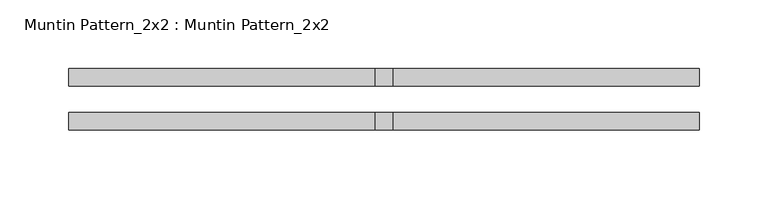
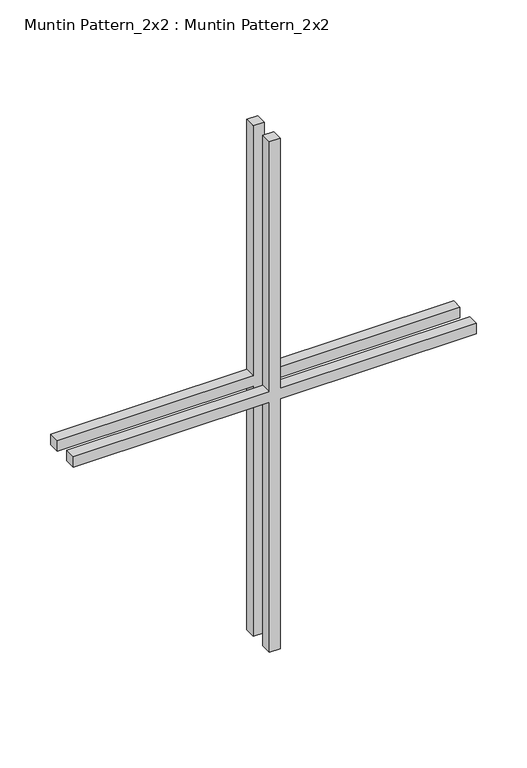
"""IFC4 building model written with IfcOpenShell, lengths in millimetres: proxy geometry, Muntin Pattern_2x2 : Muntin Pattern_2x2."""

import ifcopenshell
import ifcopenshell.guid

model = None  # the IFC model being written
_history = None  # IfcOwnerHistory: only IFC2X3 demands one
_inside = {}  # id of a spatial element -> (the spatial element, [elements in it])
_under = {}  # id of a project, library or spatial element -> (it, [spatial elements below it])
_declared = {}  # id of a project -> (the project, [libraries it declares])
_typed = {}  # id of a type object -> (the type object, [elements of that type])
_made_of = {}  # id of a material, layer set ... -> (it, [elements and type objects made of it])


def new_model(schema):
    """Start an empty IFC model of exactly this schema.

    Asked for "IFC4X3", IfcOpenShell would pick the latest addendum, in which some entities
    have other attributes; the version numbers below select the first issue.
    IFC2X3 requires an IfcOwnerHistory on every rooted entity: one is made here for all.
    """
    global model, _history
    if schema == "IFC4X3":
        model = ifcopenshell.file(schema_version=(4, 3, 0, 0))
    else:
        model = ifcopenshell.file(schema=schema)
    _inside.clear()
    _under.clear()
    _declared.clear()
    _typed.clear()
    _made_of.clear()
    _history = None
    if model.schema == "IFC2X3":
        org = make("IfcOrganization", Name="unknown")
        user = make(
            "IfcPersonAndOrganization",
            ThePerson=make("IfcPerson", FamilyName="unknown"),
            TheOrganization=org,
        )
        app = make(
            "IfcApplication",
            ApplicationDeveloper=org,
            Version="unknown",
            ApplicationFullName="unknown",
            ApplicationIdentifier="unknown",
        )
        _history = make(
            "IfcOwnerHistory",
            OwningUser=user,
            OwningApplication=app,
            ChangeAction="ADDED",
            CreationDate=0,
        )
    return model


def make(cls, **values):
    """One entity of the class cls with the attributes given. An attribute that is None is left unset."""
    return model.create_entity(
        cls, **{name: value for name, value in values.items() if value is not None}
    )


def rooted(cls, **values):
    """An entity with a GlobalId (a new one), such as an element, a storey or a relation."""
    return make(cls, GlobalId=ifcopenshell.guid.new(), OwnerHistory=_history, **values)


def si_unit(unit_type, name, prefix=None):
    """IfcSIUnit, for example si_unit("LENGTHUNIT", "METRE", prefix="MILLI")."""
    return make("IfcSIUnit", UnitType=unit_type, Prefix=prefix, Name=name)


def assignment(units):
    """IfcUnitAssignment: the units of a project."""
    return None if units is None else make("IfcUnitAssignment", Units=units)


def point(xyz):
    """IfcCartesianPoint."""
    return None if xyz is None else make("IfcCartesianPoint", Coordinates=xyz)


def direction(xyz):
    """IfcDirection."""
    return None if xyz is None else make("IfcDirection", DirectionRatios=xyz)


def frame(location, z_axis=None, x_axis=None):
    """IfcAxis2Placement3D, a coordinate frame: its origin and axes. An axis left out is left unset."""
    return make(
        "IfcAxis2Placement3D",
        Location=point(location),
        Axis=direction(z_axis),
        RefDirection=direction(x_axis),
    )


def origin():
    """The frame at (0, 0, 0) with its axes left unset."""
    return frame((0.0, 0.0, 0.0))


def place(relative_to, where):
    """IfcLocalPlacement: puts the frame where relative to a parent placement (None: the world)."""
    return make(
        "IfcLocalPlacement", PlacementRelTo=relative_to, RelativePlacement=where
    )


def context(
    kind, dimensions, precision=None, world=None, true_north=None, identifier=None
):
    """IfcGeometricRepresentationContext, for example the 3D "Model" context."""
    return make(
        "IfcGeometricRepresentationContext",
        ContextIdentifier=identifier,
        ContextType=kind,
        CoordinateSpaceDimension=dimensions,
        Precision=precision,
        WorldCoordinateSystem=world,
        TrueNorth=true_north,
    )


def project(units=None, contexts=None):
    """IfcProject with its units and contexts."""
    return rooted(
        "IfcProject",
        Name="project",
        RepresentationContexts=contexts,
        UnitsInContext=assignment(units),
    )


def spatial(cls, under=None, at=None, **own):
    """A site, building, storey or space (cls), placed at a placement, below another one or the project."""
    s = rooted(cls, ObjectPlacement=at, **own)
    if under is not None:
        _under.setdefault(under.id(), (under, []))[1].append(s)
    return s


def polyline(points):
    """IfcPolyline through the points."""
    return make("IfcPolyline", Points=[point(p) for p in points])


def outline(outer, holes=None, kind="AREA"):
    """IfcArbitraryClosedProfileDef: a profile drawn as a closed curve; with holes, ...WithVoids."""
    if holes is None:
        return make("IfcArbitraryClosedProfileDef", ProfileType=kind, OuterCurve=outer)
    return make(
        "IfcArbitraryProfileDefWithVoids",
        ProfileType=kind,
        OuterCurve=outer,
        InnerCurves=holes,
    )


def extrude(swept, where, along, depth):
    """IfcExtrudedAreaSolid: the profile swept, set in the frame where, extruded along a direction by depth."""
    return make(
        "IfcExtrudedAreaSolid",
        SweptArea=swept,
        Position=where,
        ExtrudedDirection=direction(along),
        Depth=depth,
    )


def shape(context_of_items, identifier, shape_type, items):
    """IfcShapeRepresentation: the items that make up one representation, for example the "Body"."""
    return make(
        "IfcShapeRepresentation",
        ContextOfItems=context_of_items,
        RepresentationIdentifier=identifier,
        RepresentationType=shape_type,
        Items=items,
    )


def source(mapping_origin, context_of_items, identifier, shape_type, items):
    """IfcRepresentationMap: a shape defined once, which mapped items show again and again."""
    return make(
        "IfcRepresentationMap",
        MappingOrigin=mapping_origin,
        MappedRepresentation=shape(context_of_items, identifier, shape_type, items),
    )


def transform(
    local_origin,
    x_axis=None,
    y_axis=None,
    z_axis=None,
    scale=None,
    scale2=None,
    scale3=None,
    uniform=True,
):
    """IfcCartesianTransformationOperator3D, or its non-uniform kind. x_axis, y_axis, z_axis: its Axis1, 2, 3."""
    if uniform:
        return make(
            "IfcCartesianTransformationOperator3D",
            Axis1=direction(x_axis),
            Axis2=direction(y_axis),
            LocalOrigin=point(local_origin),
            Scale=scale,
            Axis3=direction(z_axis),
        )
    return make(
        "IfcCartesianTransformationOperator3DnonUniform",
        Axis1=direction(x_axis),
        Axis2=direction(y_axis),
        LocalOrigin=point(local_origin),
        Scale=scale,
        Axis3=direction(z_axis),
        Scale2=scale2,
        Scale3=scale3,
    )


def mapped(mapping_source, mapping_target):
    """IfcMappedItem: shows the shape of a source again, moved by a transform."""
    return make(
        "IfcMappedItem", MappingSource=mapping_source, MappingTarget=mapping_target
    )


def made_of(thing, what):
    """Note that an element or type object is made of a material, layer set ...; save() writes the relation."""
    if what is not None:
        _made_of.setdefault(what.id(), (what, []))[1].append(thing)
    return thing


def element(
    cls,
    number,
    at=None,
    inside=None,
    cuts=None,
    type_object=None,
    material=None,
    context=None,
    identifier="Body",
    shape_type=None,
    held_by="IfcProductDefinitionShape",
    body=None,
    shapes=None,
    **own,
):
    """One element of the class cls, such as IfcWall. Its Tag is "e" and its number.

    at: its placement. inside: the storey or other place that contains it. cuts: it is an
    opening in that element (IfcRelVoidsElement). A single representation is given by context,
    identifier, shape_type and body (its items); several are given by shapes. held_by: the class
    of the entity that holds the representations. save() writes the other relations.
    """
    e = rooted(cls, Tag="e%d" % number, ObjectPlacement=at, **own)
    if body is not None:
        shapes = [shape(context, identifier, shape_type, body)]
    if shapes is not None:
        e.Representation = make(held_by, Representations=shapes)
    if inside is not None:
        _inside.setdefault(inside.id(), (inside, []))[1].append(e)
    if cuts is not None:
        rooted(
            "IfcRelVoidsElement", RelatingBuildingElement=cuts, RelatedOpeningElement=e
        )
    if type_object is not None:
        _typed.setdefault(type_object.id(), (type_object, []))[1].append(e)
    return made_of(e, material)


def aggregate(whole, parts):
    """IfcRelAggregates: a whole, such as a stair, and the parts it consists of."""
    return rooted("IfcRelAggregates", RelatingObject=whole, RelatedObjects=parts)


def save(model, path):
    """Write the relations noted so far, then the file.

    IfcRelAggregates (storeys below a building ...), IfcRelContainedInSpatialStructure (elements
    in a storey), IfcRelDefinesByType, IfcRelAssociatesMaterial and IfcRelDeclares: one each for
    every whole, place, type object, material and project.
    """
    for whole, parts in _under.values():
        aggregate(whole, parts)
    for where, things in _inside.values():
        rooted(
            "IfcRelContainedInSpatialStructure",
            RelatedElements=things,
            RelatingStructure=where,
        )
    for kind, things in _typed.values():
        rooted("IfcRelDefinesByType", RelatedObjects=things, RelatingType=kind)
    for what, things in _made_of.values():
        rooted("IfcRelAssociatesMaterial", RelatedObjects=things, RelatingMaterial=what)
    for by, libraries in _declared.values():
        rooted("IfcRelDeclares", RelatingContext=by, RelatedDefinitions=libraries)
    model.write(path)


def muntin_pattern_2x2_muntin_pattern_2x2_32a917e4(model_context):
    return source(origin(), model_context, "Body", "SweptSolid", [
        extrude(outline(polyline([(312.7375, -6.35), (312.7375, -228.6), (300.0375, -228.6), (300.0375, -6.35), (0.0, -6.35), (0.0, 6.35), (300.0375, 6.35), (300.0375, 228.6), (312.7375, 228.6), (312.7375, 6.35), (612.775, 6.35), (612.775, -6.35), (312.7375, -6.35)])), frame((0.0, -22.225, 0.0), z_axis=(0.0, 1.0, 0.0), x_axis=(0.0, 0.0, 1.0)), (0.0, 0.0, 1.0), 12.7),
        extrude(outline(polyline([(312.7375, -6.35), (312.7375, -228.6), (300.0375, -228.6), (300.0375, -6.35), (0.0, -6.35), (0.0, 6.35), (300.0375, 6.35), (300.0375, 228.6), (312.7375, 228.6), (312.7375, 6.35), (612.775, 6.35), (612.775, -6.35), (312.7375, -6.35)])), frame((0.0, 9.525, 0.0), z_axis=(0.0, 1.0, 0.0), x_axis=(0.0, 0.0, 1.0)), (0.0, 0.0, 1.0), 12.7),
    ])


if __name__ == "__main__":
    model = new_model("IFC4")
    model_context = context("Model", 3, world=origin())
    ifc_project = project(units=[si_unit("LENGTHUNIT", "METRE", prefix="MILLI")], contexts=[model_context])
    site = spatial("IfcSite", under=ifc_project)
    building = spatial("IfcBuilding", under=site)
    placement = place(None, origin())
    muntin_pattern_2x2_muntin_pattern_2x2_shape = muntin_pattern_2x2_muntin_pattern_2x2_32a917e4(model_context)
    element("IfcBuildingElementProxy", 1, Name="Muntin Pattern_2x2 : Muntin Pattern_2x2", ObjectType="Muntin Pattern_2x2 : Muntin Pattern_2x2", at=placement, inside=building, context=model_context, shape_type="MappedRepresentation", body=[
        mapped(muntin_pattern_2x2_muntin_pattern_2x2_shape, transform((0.0, 0.0, 0.0), x_axis=(1.0, 0.0, 0.0), y_axis=(0.0, 1.0, 0.0), z_axis=(0.0, 0.0, 1.0))),
    ])
    save(model, "model.ifc")

# Revit data of these elements
# Type "Muntin Pattern_2x2 : Muntin Pattern_2x2"
#   Width [instance default] = 4' - 0"
#   Thickness = 0' - 0 1/2"
#   Height [instance default] = 4' - 0"
#   Distance = 0' - 0 3/4"
#   Interior Material [instance default] = none
#   Exterior Material [instance default] = none
#   Default Elevation = 0
# Element 1 (IfcBuildingElementProxy, "Muntin Pattern_2x2 : Muntin Pattern_2x2")
#   Width = 1' - 6"
#   Height = 2' - 0 1/8"
#   Interior Material = Wood - Stained
#   Exterior Material = Clad - White
#   Materials on its faces: "Clad - White", "Wood - Stained"
# Materials
#   "Clad - White": class "Wood", colour RGB 242 242 238, transparency 0, Cost = 0
#   "Wood - Stained": class "Wood", colour RGB 224 178 126, transparency 0, Cost = 0
